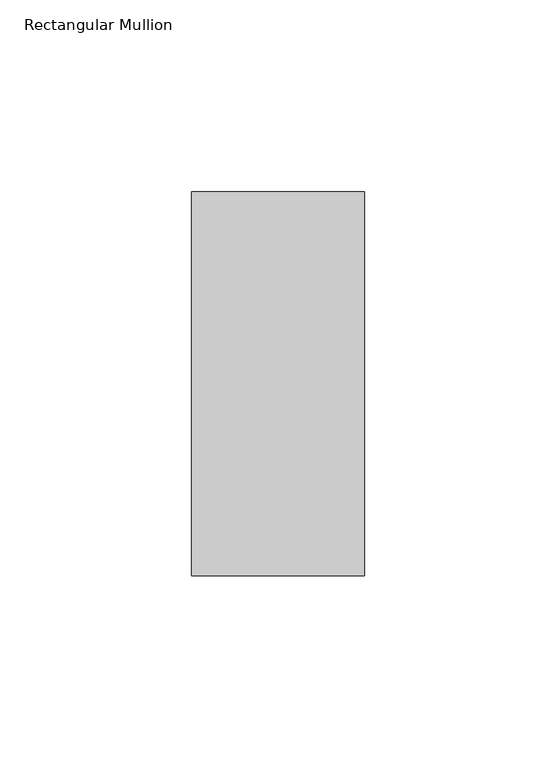
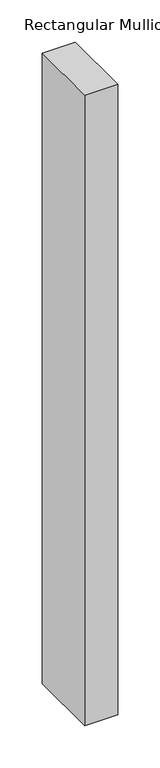
"""IFC4 building model written with IfcOpenShell, lengths in millimetres: member geometry, Rectangular Mullion : 알루미늄_Rectangular Cap_100 x 45."""

import ifcopenshell
import ifcopenshell.guid

model = None  # the IFC model being written
_history = None  # IfcOwnerHistory: only IFC2X3 demands one
_inside = {}  # id of a spatial element -> (the spatial element, [elements in it])
_under = {}  # id of a project, library or spatial element -> (it, [spatial elements below it])
_declared = {}  # id of a project -> (the project, [libraries it declares])
_typed = {}  # id of a type object -> (the type object, [elements of that type])
_made_of = {}  # id of a material, layer set ... -> (it, [elements and type objects made of it])


def new_model(schema):
    """Start an empty IFC model of exactly this schema.

    Asked for "IFC4X3", IfcOpenShell would pick the latest addendum, in which some entities
    have other attributes; the version numbers below select the first issue.
    IFC2X3 requires an IfcOwnerHistory on every rooted entity: one is made here for all.
    """
    global model, _history
    if schema == "IFC4X3":
        model = ifcopenshell.file(schema_version=(4, 3, 0, 0))
    else:
        model = ifcopenshell.file(schema=schema)
    _inside.clear()
    _under.clear()
    _declared.clear()
    _typed.clear()
    _made_of.clear()
    _history = None
    if model.schema == "IFC2X3":
        org = make("IfcOrganization", Name="unknown")
        user = make(
            "IfcPersonAndOrganization",
            ThePerson=make("IfcPerson", FamilyName="unknown"),
            TheOrganization=org,
        )
        app = make(
            "IfcApplication",
            ApplicationDeveloper=org,
            Version="unknown",
            ApplicationFullName="unknown",
            ApplicationIdentifier="unknown",
        )
        _history = make(
            "IfcOwnerHistory",
            OwningUser=user,
            OwningApplication=app,
            ChangeAction="ADDED",
            CreationDate=0,
        )
    return model


def make(cls, **values):
    """One entity of the class cls with the attributes given. An attribute that is None is left unset."""
    return model.create_entity(
        cls, **{name: value for name, value in values.items() if value is not None}
    )


def rooted(cls, **values):
    """An entity with a GlobalId (a new one), such as an element, a storey or a relation."""
    return make(cls, GlobalId=ifcopenshell.guid.new(), OwnerHistory=_history, **values)


def si_unit(unit_type, name, prefix=None):
    """IfcSIUnit, for example si_unit("LENGTHUNIT", "METRE", prefix="MILLI")."""
    return make("IfcSIUnit", UnitType=unit_type, Prefix=prefix, Name=name)


def assignment(units):
    """IfcUnitAssignment: the units of a project."""
    return None if units is None else make("IfcUnitAssignment", Units=units)


def point(xyz):
    """IfcCartesianPoint."""
    return None if xyz is None else make("IfcCartesianPoint", Coordinates=xyz)


def direction(xyz):
    """IfcDirection."""
    return None if xyz is None else make("IfcDirection", DirectionRatios=xyz)


def frame(location, z_axis=None, x_axis=None):
    """IfcAxis2Placement3D, a coordinate frame: its origin and axes. An axis left out is left unset."""
    return make(
        "IfcAxis2Placement3D",
        Location=point(location),
        Axis=direction(z_axis),
        RefDirection=direction(x_axis),
    )


def origin():
    """The frame at (0, 0, 0) with its axes left unset."""
    return frame((0.0, 0.0, 0.0))


def place(relative_to, where):
    """IfcLocalPlacement: puts the frame where relative to a parent placement (None: the world)."""
    return make(
        "IfcLocalPlacement", PlacementRelTo=relative_to, RelativePlacement=where
    )


def context(
    kind, dimensions, precision=None, world=None, true_north=None, identifier=None
):
    """IfcGeometricRepresentationContext, for example the 3D "Model" context."""
    return make(
        "IfcGeometricRepresentationContext",
        ContextIdentifier=identifier,
        ContextType=kind,
        CoordinateSpaceDimension=dimensions,
        Precision=precision,
        WorldCoordinateSystem=world,
        TrueNorth=true_north,
    )


def project(units=None, contexts=None):
    """IfcProject with its units and contexts."""
    return rooted(
        "IfcProject",
        Name="project",
        RepresentationContexts=contexts,
        UnitsInContext=assignment(units),
    )


def spatial(cls, under=None, at=None, **own):
    """A site, building, storey or space (cls), placed at a placement, below another one or the project."""
    s = rooted(cls, ObjectPlacement=at, **own)
    if under is not None:
        _under.setdefault(under.id(), (under, []))[1].append(s)
    return s


def polyline(points):
    """IfcPolyline through the points."""
    return make("IfcPolyline", Points=[point(p) for p in points])


def outline(outer, holes=None, kind="AREA"):
    """IfcArbitraryClosedProfileDef: a profile drawn as a closed curve; with holes, ...WithVoids."""
    if holes is None:
        return make("IfcArbitraryClosedProfileDef", ProfileType=kind, OuterCurve=outer)
    return make(
        "IfcArbitraryProfileDefWithVoids",
        ProfileType=kind,
        OuterCurve=outer,
        InnerCurves=holes,
    )


def extrude(swept, where, along, depth):
    """IfcExtrudedAreaSolid: the profile swept, set in the frame where, extruded along a direction by depth."""
    return make(
        "IfcExtrudedAreaSolid",
        SweptArea=swept,
        Position=where,
        ExtrudedDirection=direction(along),
        Depth=depth,
    )


def shape(context_of_items, identifier, shape_type, items):
    """IfcShapeRepresentation: the items that make up one representation, for example the "Body"."""
    return make(
        "IfcShapeRepresentation",
        ContextOfItems=context_of_items,
        RepresentationIdentifier=identifier,
        RepresentationType=shape_type,
        Items=items,
    )


def source(mapping_origin, context_of_items, identifier, shape_type, items):
    """IfcRepresentationMap: a shape defined once, which mapped items show again and again."""
    return make(
        "IfcRepresentationMap",
        MappingOrigin=mapping_origin,
        MappedRepresentation=shape(context_of_items, identifier, shape_type, items),
    )


def transform(
    local_origin,
    x_axis=None,
    y_axis=None,
    z_axis=None,
    scale=None,
    scale2=None,
    scale3=None,
    uniform=True,
):
    """IfcCartesianTransformationOperator3D, or its non-uniform kind. x_axis, y_axis, z_axis: its Axis1, 2, 3."""
    if uniform:
        return make(
            "IfcCartesianTransformationOperator3D",
            Axis1=direction(x_axis),
            Axis2=direction(y_axis),
            LocalOrigin=point(local_origin),
            Scale=scale,
            Axis3=direction(z_axis),
        )
    return make(
        "IfcCartesianTransformationOperator3DnonUniform",
        Axis1=direction(x_axis),
        Axis2=direction(y_axis),
        LocalOrigin=point(local_origin),
        Scale=scale,
        Axis3=direction(z_axis),
        Scale2=scale2,
        Scale3=scale3,
    )


def mapped(mapping_source, mapping_target):
    """IfcMappedItem: shows the shape of a source again, moved by a transform."""
    return make(
        "IfcMappedItem", MappingSource=mapping_source, MappingTarget=mapping_target
    )


def made_of(thing, what):
    """Note that an element or type object is made of a material, layer set ...; save() writes the relation."""
    if what is not None:
        _made_of.setdefault(what.id(), (what, []))[1].append(thing)
    return thing


def element(
    cls,
    number,
    at=None,
    inside=None,
    cuts=None,
    type_object=None,
    material=None,
    context=None,
    identifier="Body",
    shape_type=None,
    held_by="IfcProductDefinitionShape",
    body=None,
    shapes=None,
    **own,
):
    """One element of the class cls, such as IfcWall. Its Tag is "e" and its number.

    at: its placement. inside: the storey or other place that contains it. cuts: it is an
    opening in that element (IfcRelVoidsElement). A single representation is given by context,
    identifier, shape_type and body (its items); several are given by shapes. held_by: the class
    of the entity that holds the representations. save() writes the other relations.
    """
    e = rooted(cls, Tag="e%d" % number, ObjectPlacement=at, **own)
    if body is not None:
        shapes = [shape(context, identifier, shape_type, body)]
    if shapes is not None:
        e.Representation = make(held_by, Representations=shapes)
    if inside is not None:
        _inside.setdefault(inside.id(), (inside, []))[1].append(e)
    if cuts is not None:
        rooted(
            "IfcRelVoidsElement", RelatingBuildingElement=cuts, RelatedOpeningElement=e
        )
    if type_object is not None:
        _typed.setdefault(type_object.id(), (type_object, []))[1].append(e)
    return made_of(e, material)


def aggregate(whole, parts):
    """IfcRelAggregates: a whole, such as a stair, and the parts it consists of."""
    return rooted("IfcRelAggregates", RelatingObject=whole, RelatedObjects=parts)


def save(model, path):
    """Write the relations noted so far, then the file.

    IfcRelAggregates (storeys below a building ...), IfcRelContainedInSpatialStructure (elements
    in a storey), IfcRelDefinesByType, IfcRelAssociatesMaterial and IfcRelDeclares: one each for
    every whole, place, type object, material and project.
    """
    for whole, parts in _under.values():
        aggregate(whole, parts)
    for where, things in _inside.values():
        rooted(
            "IfcRelContainedInSpatialStructure",
            RelatedElements=things,
            RelatingStructure=where,
        )
    for kind, things in _typed.values():
        rooted("IfcRelDefinesByType", RelatedObjects=things, RelatingType=kind)
    for what, things in _made_of.values():
        rooted("IfcRelAssociatesMaterial", RelatedObjects=things, RelatingMaterial=what)
    for by, libraries in _declared.values():
        rooted("IfcRelDeclares", RelatingContext=by, RelatedDefinitions=libraries)
    model.write(path)


def rectangular_mullion_5bb1590a(model_context):
    return source(origin(), model_context, "Body", "SweptSolid", [
        extrude(outline(polyline([(22.5, 50.0), (22.5, -50.0), (-22.5, -50.0), (-22.5, 50.0), (22.5, 50.0)])), frame((0.0, 0.0, -910.0), z_axis=(0.0, 0.0, 1.0), x_axis=(1.0, 0.0, 0.0)), (0.0, 0.0, 1.0), 910.0),
    ])


if __name__ == "__main__":
    model = new_model("IFC4")
    model_context = context("Model", 3, world=origin())
    ifc_project = project(units=[si_unit("LENGTHUNIT", "METRE", prefix="MILLI")], contexts=[model_context])
    site = spatial("IfcSite", under=ifc_project)
    building = spatial("IfcBuilding", under=site)
    placement = place(None, origin())
    rectangular_mullion_shape = rectangular_mullion_5bb1590a(model_context)
    element("IfcMember", 1, ObjectType="Rectangular Mullion : 알루미늄_Rectangular Cap_100 x 45", at=placement, inside=building, context=model_context, shape_type="MappedRepresentation", body=[
        mapped(rectangular_mullion_shape, transform((0.0, 0.0, 0.0), x_axis=(1.0, 0.0, 0.0), y_axis=(0.0, 1.0, 0.0), z_axis=(0.0, 0.0, 1.0))),
    ])
    save(model, "model.ifc")

# Revit data of these elements
# Type "Rectangular Mullion : 알루미늄_Rectangular Cap_100 x 45"
#   built-in parameter 1007304 = 0.328084 (stored number, unit not read)
#   built-in parameter 1007301 = 0.0738189 (stored number, unit not read)
#   built-in parameter 1007300 = 0.0738189 (stored number, unit not read)
# Element 1 (IfcMember, "Rectangular Mullion : 알루미늄_Rectangular Cap_100 x 45")
#   Materials on its faces: "00_Metal_Stainless Steel"
# Materials
#   "00_Metal_Stainless Steel": class "Metal", colour RGB 148 148 148, transparency 0, Description = "Steel", Cost = 0
